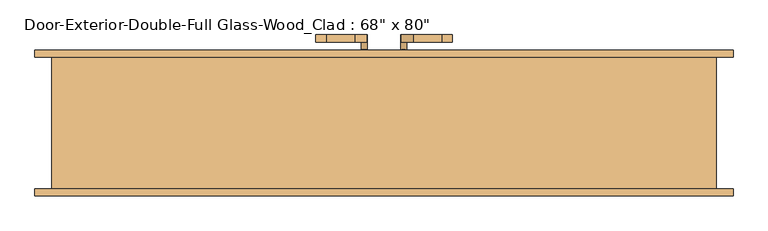
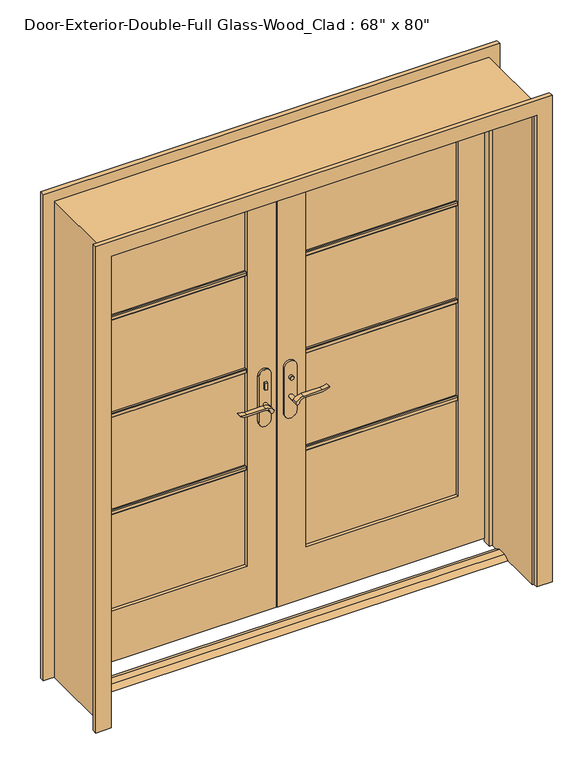
"""IFC4 building model written with IfcOpenShell, lengths in millimetres: door geometry."""

import ifcopenshell
import ifcopenshell.guid

model = None  # the IFC model being written
_history = None  # IfcOwnerHistory: only IFC2X3 demands one
_inside = {}  # id of a spatial element -> (the spatial element, [elements in it])
_under = {}  # id of a project, library or spatial element -> (it, [spatial elements below it])
_declared = {}  # id of a project -> (the project, [libraries it declares])
_typed = {}  # id of a type object -> (the type object, [elements of that type])
_made_of = {}  # id of a material, layer set ... -> (it, [elements and type objects made of it])


def new_model(schema):
    """Start an empty IFC model of exactly this schema.

    Asked for "IFC4X3", IfcOpenShell would pick the latest addendum, in which some entities
    have other attributes; the version numbers below select the first issue.
    IFC2X3 requires an IfcOwnerHistory on every rooted entity: one is made here for all.
    """
    global model, _history
    if schema == "IFC4X3":
        model = ifcopenshell.file(schema_version=(4, 3, 0, 0))
    else:
        model = ifcopenshell.file(schema=schema)
    _inside.clear()
    _under.clear()
    _declared.clear()
    _typed.clear()
    _made_of.clear()
    _history = None
    if model.schema == "IFC2X3":
        org = make("IfcOrganization", Name="unknown")
        user = make(
            "IfcPersonAndOrganization",
            ThePerson=make("IfcPerson", FamilyName="unknown"),
            TheOrganization=org,
        )
        app = make(
            "IfcApplication",
            ApplicationDeveloper=org,
            Version="unknown",
            ApplicationFullName="unknown",
            ApplicationIdentifier="unknown",
        )
        _history = make(
            "IfcOwnerHistory",
            OwningUser=user,
            OwningApplication=app,
            ChangeAction="ADDED",
            CreationDate=0,
        )
    return model


def make(cls, **values):
    """One entity of the class cls with the attributes given. An attribute that is None is left unset."""
    return model.create_entity(
        cls, **{name: value for name, value in values.items() if value is not None}
    )


def rooted(cls, **values):
    """An entity with a GlobalId (a new one), such as an element, a storey or a relation."""
    return make(cls, GlobalId=ifcopenshell.guid.new(), OwnerHistory=_history, **values)


def si_unit(unit_type, name, prefix=None):
    """IfcSIUnit, for example si_unit("LENGTHUNIT", "METRE", prefix="MILLI")."""
    return make("IfcSIUnit", UnitType=unit_type, Prefix=prefix, Name=name)


def assignment(units):
    """IfcUnitAssignment: the units of a project."""
    return None if units is None else make("IfcUnitAssignment", Units=units)


def point(xyz):
    """IfcCartesianPoint."""
    return None if xyz is None else make("IfcCartesianPoint", Coordinates=xyz)


def direction(xyz):
    """IfcDirection."""
    return None if xyz is None else make("IfcDirection", DirectionRatios=xyz)


def frame(location, z_axis=None, x_axis=None):
    """IfcAxis2Placement3D, a coordinate frame: its origin and axes. An axis left out is left unset."""
    return make(
        "IfcAxis2Placement3D",
        Location=point(location),
        Axis=direction(z_axis),
        RefDirection=direction(x_axis),
    )


def frame_2d(location, x_axis=None):
    """IfcAxis2Placement2D, a coordinate frame in the plane: its origin and x axis."""
    return make(
        "IfcAxis2Placement2D", Location=point(location), RefDirection=direction(x_axis)
    )


def origin():
    """The frame at (0, 0, 0) with its axes left unset."""
    return frame((0.0, 0.0, 0.0))


def place(relative_to, where):
    """IfcLocalPlacement: puts the frame where relative to a parent placement (None: the world)."""
    return make(
        "IfcLocalPlacement", PlacementRelTo=relative_to, RelativePlacement=where
    )


def context(
    kind, dimensions, precision=None, world=None, true_north=None, identifier=None
):
    """IfcGeometricRepresentationContext, for example the 3D "Model" context."""
    return make(
        "IfcGeometricRepresentationContext",
        ContextIdentifier=identifier,
        ContextType=kind,
        CoordinateSpaceDimension=dimensions,
        Precision=precision,
        WorldCoordinateSystem=world,
        TrueNorth=true_north,
    )


def project(units=None, contexts=None):
    """IfcProject with its units and contexts."""
    return rooted(
        "IfcProject",
        Name="project",
        RepresentationContexts=contexts,
        UnitsInContext=assignment(units),
    )


def spatial(cls, under=None, at=None, **own):
    """A site, building, storey or space (cls), placed at a placement, below another one or the project."""
    s = rooted(cls, ObjectPlacement=at, **own)
    if under is not None:
        _under.setdefault(under.id(), (under, []))[1].append(s)
    return s


def polyline(points):
    """IfcPolyline through the points."""
    return make("IfcPolyline", Points=[point(p) for p in points])


def circle_curve(where, radius):
    """IfcCircle in the frame where."""
    return make("IfcCircle", Position=where, Radius=radius)


def trimmed(basis, trim1, trim2, sense, master):
    """IfcTrimmedCurve: the piece of a basis curve between two trims."""
    return make(
        "IfcTrimmedCurve",
        BasisCurve=basis,
        Trim1=trim1,
        Trim2=trim2,
        SenseAgreement=sense,
        MasterRepresentation=master,
    )


def segment(curve, same_sense, transition):
    """IfcCompositeCurveSegment."""
    return make(
        "IfcCompositeCurveSegment",
        Transition=transition,
        SameSense=same_sense,
        ParentCurve=curve,
    )


def composite_curve(segments, self_intersect=None):
    """IfcCompositeCurve: segments joined end to end."""
    return make("IfcCompositeCurve", Segments=segments, SelfIntersect=self_intersect)


def outline(outer, holes=None, kind="AREA"):
    """IfcArbitraryClosedProfileDef: a profile drawn as a closed curve; with holes, ...WithVoids."""
    if holes is None:
        return make("IfcArbitraryClosedProfileDef", ProfileType=kind, OuterCurve=outer)
    return make(
        "IfcArbitraryProfileDefWithVoids",
        ProfileType=kind,
        OuterCurve=outer,
        InnerCurves=holes,
    )


def extrude(swept, where, along, depth):
    """IfcExtrudedAreaSolid: the profile swept, set in the frame where, extruded along a direction by depth."""
    return make(
        "IfcExtrudedAreaSolid",
        SweptArea=swept,
        Position=where,
        ExtrudedDirection=direction(along),
        Depth=depth,
    )


def faces_of(points, faces, orient=None, outer=None):
    """IfcFace entities. A face is a list of loops; a loop is a list of indices into points, from 0.

    orient and outer hold one flag for each loop. By default every Orientation is true, the
    first loop of a face is its IfcFaceOuterBound and the others are IfcFaceBound.
    """
    made = []
    for i, loops in enumerate(faces):
        bounds = []
        for j, loop in enumerate(loops):
            is_outer = j == 0 if outer is None else outer[i][j]
            bounds.append(
                make(
                    "IfcFaceOuterBound" if is_outer else "IfcFaceBound",
                    Bound=make("IfcPolyLoop", Polygon=[points[k] for k in loop]),
                    Orientation=True if orient is None else orient[i][j],
                )
            )
        made.append(make("IfcFace", Bounds=bounds))
    return made


def faceted_brep(points, faces, orient=None, outer=None, voids=None):
    """IfcFacetedBrep: a solid bounded by flat faces; with voids (closed shells), ...WithVoids."""
    shared = [point(p) for p in points]
    hull = make("IfcClosedShell", CfsFaces=faces_of(shared, faces, orient, outer))
    if voids is None:
        return make("IfcFacetedBrep", Outer=hull)
    return make(
        "IfcFacetedBrepWithVoids",
        Outer=hull,
        Voids=[
            make(cls, CfsFaces=faces_of(shared, fs, o, b)) for cls, fs, o, b in voids
        ],
    )


def shape(context_of_items, identifier, shape_type, items):
    """IfcShapeRepresentation: the items that make up one representation, for example the "Body"."""
    return make(
        "IfcShapeRepresentation",
        ContextOfItems=context_of_items,
        RepresentationIdentifier=identifier,
        RepresentationType=shape_type,
        Items=items,
    )


def source(mapping_origin, context_of_items, identifier, shape_type, items):
    """IfcRepresentationMap: a shape defined once, which mapped items show again and again."""
    return make(
        "IfcRepresentationMap",
        MappingOrigin=mapping_origin,
        MappedRepresentation=shape(context_of_items, identifier, shape_type, items),
    )


def transform(
    local_origin,
    x_axis=None,
    y_axis=None,
    z_axis=None,
    scale=None,
    scale2=None,
    scale3=None,
    uniform=True,
):
    """IfcCartesianTransformationOperator3D, or its non-uniform kind. x_axis, y_axis, z_axis: its Axis1, 2, 3."""
    if uniform:
        return make(
            "IfcCartesianTransformationOperator3D",
            Axis1=direction(x_axis),
            Axis2=direction(y_axis),
            LocalOrigin=point(local_origin),
            Scale=scale,
            Axis3=direction(z_axis),
        )
    return make(
        "IfcCartesianTransformationOperator3DnonUniform",
        Axis1=direction(x_axis),
        Axis2=direction(y_axis),
        LocalOrigin=point(local_origin),
        Scale=scale,
        Axis3=direction(z_axis),
        Scale2=scale2,
        Scale3=scale3,
    )


def mapped(mapping_source, mapping_target):
    """IfcMappedItem: shows the shape of a source again, moved by a transform."""
    return make(
        "IfcMappedItem", MappingSource=mapping_source, MappingTarget=mapping_target
    )


def made_of(thing, what):
    """Note that an element or type object is made of a material, layer set ...; save() writes the relation."""
    if what is not None:
        _made_of.setdefault(what.id(), (what, []))[1].append(thing)
    return thing


def element(
    cls,
    number,
    at=None,
    inside=None,
    cuts=None,
    type_object=None,
    material=None,
    context=None,
    identifier="Body",
    shape_type=None,
    held_by="IfcProductDefinitionShape",
    body=None,
    shapes=None,
    **own,
):
    """One element of the class cls, such as IfcWall. Its Tag is "e" and its number.

    at: its placement. inside: the storey or other place that contains it. cuts: it is an
    opening in that element (IfcRelVoidsElement). A single representation is given by context,
    identifier, shape_type and body (its items); several are given by shapes. held_by: the class
    of the entity that holds the representations. save() writes the other relations.
    """
    e = rooted(cls, Tag="e%d" % number, ObjectPlacement=at, **own)
    if body is not None:
        shapes = [shape(context, identifier, shape_type, body)]
    if shapes is not None:
        e.Representation = make(held_by, Representations=shapes)
    if inside is not None:
        _inside.setdefault(inside.id(), (inside, []))[1].append(e)
    if cuts is not None:
        rooted(
            "IfcRelVoidsElement", RelatingBuildingElement=cuts, RelatedOpeningElement=e
        )
    if type_object is not None:
        _typed.setdefault(type_object.id(), (type_object, []))[1].append(e)
    return made_of(e, material)


def aggregate(whole, parts):
    """IfcRelAggregates: a whole, such as a stair, and the parts it consists of."""
    return rooted("IfcRelAggregates", RelatingObject=whole, RelatedObjects=parts)


def save(model, path):
    """Write the relations noted so far, then the file.

    IfcRelAggregates (storeys below a building ...), IfcRelContainedInSpatialStructure (elements
    in a storey), IfcRelDefinesByType, IfcRelAssociatesMaterial and IfcRelDeclares: one each for
    every whole, place, type object, material and project.
    """
    for whole, parts in _under.values():
        aggregate(whole, parts)
    for where, things in _inside.values():
        rooted(
            "IfcRelContainedInSpatialStructure",
            RelatedElements=things,
            RelatingStructure=where,
        )
    for kind, things in _typed.values():
        rooted("IfcRelDefinesByType", RelatedObjects=things, RelatingType=kind)
    for what, things in _made_of.values():
        rooted("IfcRelAssociatesMaterial", RelatedObjects=things, RelatingMaterial=what)
    for by, libraries in _declared.values():
        rooted("IfcRelDeclares", RelatingContext=by, RelatedDefinitions=libraries)
    model.write(path)


def door_e0419d21(model_context):
    return source(origin(), model_context, "Body", "SolidModel", [
        extrude(outline(polyline([(19.05, 12.7), (53.975, 12.7), (79.375, 0.0), (-6.35, 0.0), (19.05, 12.7)])), frame((-863.6, 0.0, 0.0), z_axis=(1.0, 0.0, 0.0), x_axis=(0.0, 1.0, 0.0)), (0.0, 0.0, 1.0), 1727.2),
        extrude(outline(polyline([(-47.4019111, 118.1125), (-57.4019111, 118.1125), (-57.4019111, 128.1125), (-47.4019111, 128.1125), (-47.4019111, 118.1125)])), frame((0.0, 0.0, 981.9), z_axis=(0.0, 0.0, 1.0), x_axis=(1.0, 0.0, 0.0)), (0.0, 0.0, 1.0), 30.0),
        extrude(outline(composite_curve([segment(trimmed(circle_curve(frame_2d((996.9, -52.4019111)), 8.0), [point((996.9, -60.4019111))], [point((996.9, -44.4019111))], False, "CARTESIAN"), True, "CONTINUOUS"), segment(trimmed(circle_curve(frame_2d((996.9, -52.4019111)), 8.0), [point((996.9, -44.4019111))], [point((996.9, -60.4019111))], False, "CARTESIAN"), True, "CONTINUOUS")], self_intersect=False)), frame((0.0, 183.0375, 0.0), z_axis=(0.0, 1.0, 0.0), x_axis=(0.0, 0.0, 1.0)), (0.0, 0.0, 1.0), 10.0),
        extrude(outline(composite_curve([segment(trimmed(circle_curve(frame_2d((897.1555521, -76.0694241)), 37.2832219), [point((919.0523287, -45.8937749))], [point((934.4, -77.7693445))], False, "CARTESIAN"), True, "CONTINUOUS"), segment(polyline([(934.4, -77.7693445), (934.4, -154.045502)]), True, "CONTINUOUS"), segment(trimmed(circle_curve(frame_2d((1017.6850638, -153.9791202)), 83.2850902), [point((934.4, -154.045502))], [point((939.4, -182.4019111))], True, "CARTESIAN"), True, "CONTINUOUS"), segment(polyline([(939.4, -182.4019111), (936.6135558, -182.4019111)]), True, "CONTINUOUS"), segment(trimmed(circle_curve(frame_2d((986.6709207, -150.4622499)), 59.3791355), [point((936.6135558, -182.4019111))], [point((927.4, -154.045502))], False, "CARTESIAN"), True, "CONTINUOUS"), segment(polyline([(927.4, -154.045502), (927.4, -77.7881013)]), True, "CONTINUOUS"), segment(trimmed(circle_curve(frame_2d((909.2738613, -77.7881013)), 18.1261387), [point((927.4, -77.7881013))], [point((914.4, -60.4019111))], True, "CARTESIAN"), True, "CONTINUOUS"), segment(trimmed(circle_curve(frame_2d((914.4, -52.4019111)), 8.0), [point((914.4, -60.4019111))], [point((919.0523287, -45.8937749))], False, "CARTESIAN"), True, "CONTINUOUS")], self_intersect=False)), frame((0.0, 78.1125, 0.0), z_axis=(0.0, 1.0, 0.0), x_axis=(0.0, 0.0, 1.0)), (0.0, 0.0, 1.0), 20.0),
        extrude(outline(composite_curve([segment(trimmed(circle_curve(frame_2d((914.4, -52.4019111)), 8.0), [point((914.3999903, -60.4019111))], [point((919.0523287, -45.8937749))], False, "CARTESIAN"), True, "CONTINUOUS"), segment(trimmed(circle_curve(frame_2d((897.1555521, -76.0694241)), 37.2832219), [point((919.0523287, -45.8937749))], [point((934.4, -77.7693445))], False, "CARTESIAN"), True, "CONTINUOUS"), segment(polyline([(934.4, -77.7693445), (934.4, -154.045502)]), True, "CONTINUOUS"), segment(trimmed(circle_curve(frame_2d((1017.6850638, -153.9791202)), 83.2850902), [point((934.4, -154.045502))], [point((939.4, -182.4019111))], True, "CARTESIAN"), True, "CONTINUOUS"), segment(polyline([(939.4, -182.4019111), (936.6135558, -182.4019111)]), True, "CONTINUOUS"), segment(trimmed(circle_curve(frame_2d((986.6709207, -150.4622499)), 59.3791355), [point((936.6135558, -182.4019111))], [point((927.4, -154.045502))], False, "CARTESIAN"), True, "CONTINUOUS"), segment(polyline([(927.4, -154.045502), (927.4, -77.788099)]), True, "CONTINUOUS"), segment(trimmed(circle_curve(frame_2d((909.2738682, -77.788099)), 18.1261318), [point((927.4, -77.788099))], [point((914.3999903, -60.4019111))], True, "CARTESIAN"), True, "CONTINUOUS")], self_intersect=False)), frame((0.0, 213.0375, 0.0), z_axis=(0.0, 1.0, 0.0), x_axis=(0.0, 0.0, 1.0)), (0.0, 0.0, 1.0), 20.0),
        extrude(outline(composite_curve([segment(trimmed(circle_curve(frame_2d((914.4, -52.4019111)), 8.0), [point((914.4, -60.4019111))], [point((914.4, -44.4019111))], False, "CARTESIAN"), True, "CONTINUOUS"), segment(trimmed(circle_curve(frame_2d((914.4, -52.4019111)), 8.0), [point((914.4, -44.4019111))], [point((914.4, -60.4019111))], False, "CARTESIAN"), True, "CONTINUOUS")], self_intersect=False)), frame((0.0, 98.1125, 0.0), z_axis=(0.0, 1.0, 0.0), x_axis=(0.0, 0.0, 1.0)), (0.0, 0.0, 1.0), 30.0),
        extrude(outline(composite_curve([segment(trimmed(circle_curve(frame_2d((914.4, -52.4019111)), 8.0), [point((914.4, -60.4019111))], [point((914.4, -44.4019111))], False, "CARTESIAN"), True, "CONTINUOUS"), segment(trimmed(circle_curve(frame_2d((914.4, -52.4019111)), 8.0), [point((914.4, -44.4019111))], [point((914.4, -60.4019111))], False, "CARTESIAN"), True, "CONTINUOUS")], self_intersect=False)), frame((0.0, 183.0375, 0.0), z_axis=(0.0, 1.0, 0.0), x_axis=(0.0, 0.0, 1.0)), (0.0, 0.0, 1.0), 30.0),
        extrude(outline(composite_curve([segment(polyline([(844.4, -27.4019111), (1039.4, -27.4019111)]), True, "CONTINUOUS"), segment(trimmed(circle_curve(frame_2d((1039.4, -52.4019111)), 25.0), [point((1039.4, -27.4019111))], [point((1039.4, -77.4019111))], False, "CARTESIAN"), True, "CONTINUOUS"), segment(polyline([(1039.4, -77.4019111), (844.4, -77.4019111)]), True, "CONTINUOUS"), segment(trimmed(circle_curve(frame_2d((844.4, -52.4019111)), 25.0), [point((844.4, -77.4019111))], [point((844.4, -27.4019111))], False, "CARTESIAN"), True, "CONTINUOUS")], self_intersect=False)), frame((0.0, 128.1125, 0.0), z_axis=(0.0, 1.0, 0.0), x_axis=(0.0, 0.0, 1.0)), (0.0, 0.0, 1.0), 10.0),
        extrude(outline(composite_curve([segment(polyline([(844.4, -27.4019111), (1039.4, -27.4019111)]), True, "CONTINUOUS"), segment(trimmed(circle_curve(frame_2d((1039.4, -52.4019111)), 25.0), [point((1039.4, -27.4019111))], [point((1039.4, -77.4019111))], False, "CARTESIAN"), True, "CONTINUOUS"), segment(polyline([(1039.4, -77.4019111), (844.4, -77.4019111)]), True, "CONTINUOUS"), segment(trimmed(circle_curve(frame_2d((844.4, -52.4019111)), 25.0), [point((844.4, -77.4019111))], [point((844.4, -27.4019111))], False, "CARTESIAN"), True, "CONTINUOUS")], self_intersect=False)), frame((0.0, 173.0375, 0.0), z_axis=(0.0, 1.0, 0.0), x_axis=(0.0, 0.0, 1.0)), (0.0, 0.0, 1.0), 10.0),
        extrude(outline(polyline([(47.3875, 193.0375), (57.3875, 193.0375), (57.3875, 183.0375), (47.3875, 183.0375), (47.3875, 193.0375)])), frame((0.0, 0.0, 981.9), z_axis=(0.0, 0.0, 1.0), x_axis=(1.0, 0.0, 0.0)), (0.0, 0.0, 1.0), 30.0),
        extrude(outline(composite_curve([segment(trimmed(circle_curve(frame_2d((996.9, 52.3875)), 8.0), [point((996.9, 60.3875))], [point((996.9, 44.3875))], False, "CARTESIAN"), True, "CONTINUOUS"), segment(trimmed(circle_curve(frame_2d((996.9, 52.3875)), 8.0), [point((996.9, 44.3875))], [point((996.9, 60.3875))], False, "CARTESIAN"), True, "CONTINUOUS")], self_intersect=False)), frame((0.0, 118.1125, 0.0), z_axis=(0.0, 1.0, 0.0), x_axis=(0.0, 0.0, 1.0)), (0.0, 0.0, 1.0), 10.0),
        extrude(outline(composite_curve([segment(trimmed(circle_curve(frame_2d((914.4, 52.3875)), 8.0), [point((919.0523287, 45.8793637))], [point((914.4, 60.3875))], False, "CARTESIAN"), True, "CONTINUOUS"), segment(trimmed(circle_curve(frame_2d((909.2738613, 77.7736901)), 18.1261387), [point((914.4, 60.3875))], [point((927.4, 77.7736901))], True, "CARTESIAN"), True, "CONTINUOUS"), segment(polyline([(927.4, 77.7736901), (927.4, 154.0310909)]), True, "CONTINUOUS"), segment(trimmed(circle_curve(frame_2d((986.6709207, 150.4478388)), 59.3791355), [point((927.4, 154.0310909))], [point((936.6135558, 182.3875))], False, "CARTESIAN"), True, "CONTINUOUS"), segment(polyline([(936.6135558, 182.3875), (939.4, 182.3875)]), True, "CONTINUOUS"), segment(trimmed(circle_curve(frame_2d((1017.6850638, 153.9647091)), 83.2850902), [point((939.4, 182.3875))], [point((934.4, 154.0310909))], True, "CARTESIAN"), True, "CONTINUOUS"), segment(polyline([(934.4, 154.0310909), (934.4, 77.7549333)]), True, "CONTINUOUS"), segment(trimmed(circle_curve(frame_2d((897.1555521, 76.0550129)), 37.2832219), [point((934.4, 77.7549333))], [point((919.0523287, 45.8793637))], False, "CARTESIAN"), True, "CONTINUOUS")], self_intersect=False)), frame((0.0, 213.0375, 0.0), z_axis=(0.0, 1.0, 0.0), x_axis=(0.0, 0.0, 1.0)), (0.0, 0.0, 1.0), 20.0),
        extrude(outline(composite_curve([segment(trimmed(circle_curve(frame_2d((909.2738682, 77.7736878)), 18.1261318), [point((914.3999903, 60.3875))], [point((927.4, 77.7736878))], True, "CARTESIAN"), True, "CONTINUOUS"), segment(polyline([(927.4, 77.7736878), (927.4, 154.0310909)]), True, "CONTINUOUS"), segment(trimmed(circle_curve(frame_2d((986.6709207, 150.4478388)), 59.3791355), [point((927.4, 154.0310909))], [point((936.6135558, 182.3875))], False, "CARTESIAN"), True, "CONTINUOUS"), segment(polyline([(936.6135558, 182.3875), (939.4, 182.3875)]), True, "CONTINUOUS"), segment(trimmed(circle_curve(frame_2d((1017.6850638, 153.9647091)), 83.2850902), [point((939.4, 182.3875))], [point((934.4, 154.0310909))], True, "CARTESIAN"), True, "CONTINUOUS"), segment(polyline([(934.4, 154.0310909), (934.4, 77.7549333)]), True, "CONTINUOUS"), segment(trimmed(circle_curve(frame_2d((897.1555521, 76.0550129)), 37.2832219), [point((934.4, 77.7549333))], [point((919.0523287, 45.8793637))], False, "CARTESIAN"), True, "CONTINUOUS"), segment(trimmed(circle_curve(frame_2d((914.4, 52.3875)), 8.0), [point((919.0523287, 45.8793637))], [point((914.3999903, 60.3875))], False, "CARTESIAN"), True, "CONTINUOUS")], self_intersect=False)), frame((0.0, 78.1125, 0.0), z_axis=(0.0, 1.0, 0.0), x_axis=(0.0, 0.0, 1.0)), (0.0, 0.0, 1.0), 20.0),
        extrude(outline(composite_curve([segment(trimmed(circle_curve(frame_2d((914.4, 52.3875)), 8.0), [point((914.4, 60.3875))], [point((914.4, 44.3875))], False, "CARTESIAN"), True, "CONTINUOUS"), segment(trimmed(circle_curve(frame_2d((914.4, 52.3875)), 8.0), [point((914.4, 44.3875))], [point((914.4, 60.3875))], False, "CARTESIAN"), True, "CONTINUOUS")], self_intersect=False)), frame((0.0, 183.0375, 0.0), z_axis=(0.0, 1.0, 0.0), x_axis=(0.0, 0.0, 1.0)), (0.0, 0.0, 1.0), 30.0),
        extrude(outline(composite_curve([segment(trimmed(circle_curve(frame_2d((914.4, 52.3875)), 8.0), [point((914.4, 60.3875))], [point((914.4, 44.3875))], False, "CARTESIAN"), True, "CONTINUOUS"), segment(trimmed(circle_curve(frame_2d((914.4, 52.3875)), 8.0), [point((914.4, 44.3875))], [point((914.4, 60.3875))], False, "CARTESIAN"), True, "CONTINUOUS")], self_intersect=False)), frame((0.0, 98.1125, 0.0), z_axis=(0.0, 1.0, 0.0), x_axis=(0.0, 0.0, 1.0)), (0.0, 0.0, 1.0), 30.0),
        extrude(outline(composite_curve([segment(trimmed(circle_curve(frame_2d((844.4, 52.3875)), 25.0), [point((844.4, 27.3875))], [point((844.4, 77.3875))], False, "CARTESIAN"), True, "CONTINUOUS"), segment(polyline([(844.4, 77.3875), (1039.4, 77.3875)]), True, "CONTINUOUS"), segment(trimmed(circle_curve(frame_2d((1039.4, 52.3875)), 25.0), [point((1039.4, 77.3875))], [point((1039.4, 27.3875))], False, "CARTESIAN"), True, "CONTINUOUS"), segment(polyline([(1039.4, 27.3875), (844.4, 27.3875)]), True, "CONTINUOUS")], self_intersect=False)), frame((0.0, 173.0375, 0.0), z_axis=(0.0, 1.0, 0.0), x_axis=(0.0, 0.0, 1.0)), (0.0, 0.0, 1.0), 10.0),
        extrude(outline(composite_curve([segment(trimmed(circle_curve(frame_2d((844.4, 52.3875)), 25.0), [point((844.4, 27.3875))], [point((844.4, 77.3875))], False, "CARTESIAN"), True, "CONTINUOUS"), segment(polyline([(844.4, 77.3875), (1039.4, 77.3875)]), True, "CONTINUOUS"), segment(trimmed(circle_curve(frame_2d((1039.4, 52.3875)), 25.0), [point((1039.4, 77.3875))], [point((1039.4, 27.3875))], False, "CARTESIAN"), True, "CONTINUOUS"), segment(polyline([(1039.4, 27.3875), (844.4, 27.3875)]), True, "CONTINUOUS")], self_intersect=False)), frame((0.0, 128.1125, 0.0), z_axis=(0.0, 1.0, 0.0), x_axis=(0.0, 0.0, 1.0)), (0.0, 0.0, 1.0), 10.0),
        extrude(outline(polyline([(152.0825, 1502.171875), (152.0825, 1483.121875), (145.7325, 1483.121875), (142.5575, 1486.296875), (142.5575, 1498.996875), (145.7325, 1502.171875), (152.0825, 1502.171875)])), frame((120.65, 0.0, 0.0), z_axis=(1.0, 0.0, 0.0), x_axis=(0.0, 1.0, 0.0)), (0.0, 0.0, 1.0), 622.3),
        extrude(outline(polyline([(152.0825, 1081.88125), (152.0825, 1062.83125), (145.7325, 1062.83125), (142.5575, 1066.00625), (142.5575, 1078.70625), (145.7325, 1081.88125), (152.0825, 1081.88125)])), frame((120.65, 0.0, 0.0), z_axis=(1.0, 0.0, 0.0), x_axis=(0.0, 1.0, 0.0)), (0.0, 0.0, 1.0), 622.3),
        extrude(outline(polyline([(152.0825, 661.590625), (152.0825, 642.540625), (145.7325, 642.540625), (142.5575, 645.715625), (142.5575, 658.415625), (145.7325, 661.590625), (152.0825, 661.590625)])), frame((120.65, 0.0, 0.0), z_axis=(1.0, 0.0, 0.0), x_axis=(0.0, 1.0, 0.0)), (0.0, 0.0, 1.0), 622.3),
        extrude(outline(polyline([(159.0675, 1502.171875), (165.4175, 1502.171875), (168.5925, 1498.996875), (168.5925, 1486.296875), (165.4175, 1483.121875), (159.0675, 1483.121875), (159.0675, 1502.171875)])), frame((-742.95, 0.0, 0.0), z_axis=(1.0, 0.0, 0.0), x_axis=(0.0, 1.0, 0.0)), (0.0, 0.0, 1.0), 622.3),
        extrude(outline(polyline([(159.0675, 1081.88125), (165.4175, 1081.88125), (168.5925, 1078.70625), (168.5925, 1066.00625), (165.4175, 1062.83125), (159.0675, 1062.83125), (159.0675, 1081.88125)])), frame((-742.95, 0.0, 0.0), z_axis=(1.0, 0.0, 0.0), x_axis=(0.0, 1.0, 0.0)), (0.0, 0.0, 1.0), 622.3),
        extrude(outline(polyline([(159.0675, 661.590625), (165.4175, 661.590625), (168.5925, 658.415625), (168.5925, 645.715625), (165.4175, 642.540625), (159.0675, 642.540625), (159.0675, 661.590625)])), frame((-742.95, 0.0, 0.0), z_axis=(1.0, 0.0, 0.0), x_axis=(0.0, 1.0, 0.0)), (0.0, 0.0, 1.0), 622.3),
        extrude(outline(polyline([(159.0675, 1502.171875), (165.4175, 1502.171875), (168.5925, 1498.996875), (168.5925, 1486.296875), (165.4175, 1483.121875), (159.0675, 1483.121875), (159.0675, 1502.171875)])), frame((120.65, 0.0, 0.0), z_axis=(1.0, 0.0, 0.0), x_axis=(0.0, 1.0, 0.0)), (0.0, 0.0, 1.0), 622.3),
        extrude(outline(polyline([(159.0675, 1081.88125), (165.4175, 1081.88125), (168.5925, 1078.70625), (168.5925, 1066.00625), (165.4175, 1062.83125), (159.0675, 1062.83125), (159.0675, 1081.88125)])), frame((120.65, 0.0, 0.0), z_axis=(1.0, 0.0, 0.0), x_axis=(0.0, 1.0, 0.0)), (0.0, 0.0, 1.0), 622.3),
        extrude(outline(polyline([(159.0675, 661.590625), (165.4175, 661.590625), (168.5925, 658.415625), (168.5925, 645.715625), (165.4175, 642.540625), (159.0675, 642.540625), (159.0675, 661.590625)])), frame((120.65, 0.0, 0.0), z_axis=(1.0, 0.0, 0.0), x_axis=(0.0, 1.0, 0.0)), (0.0, 0.0, 1.0), 622.3),
        extrude(outline(polyline([(152.0825, 1502.171875), (152.0825, 1483.121875), (145.7325, 1483.121875), (142.5575, 1486.296875), (142.5575, 1498.996875), (145.7325, 1502.171875), (152.0825, 1502.171875)])), frame((-742.95, 0.0, 0.0), z_axis=(1.0, 0.0, 0.0), x_axis=(0.0, 1.0, 0.0)), (0.0, 0.0, 1.0), 622.3),
        extrude(outline(polyline([(152.0825, 1081.88125), (152.0825, 1062.83125), (145.7325, 1062.83125), (142.5575, 1066.00625), (142.5575, 1078.70625), (145.7325, 1081.88125), (152.0825, 1081.88125)])), frame((-742.95, 0.0, 0.0), z_axis=(1.0, 0.0, 0.0), x_axis=(0.0, 1.0, 0.0)), (0.0, 0.0, 1.0), 622.3),
        extrude(outline(polyline([(152.0825, 661.590625), (152.0825, 642.540625), (145.7325, 642.540625), (142.5575, 645.715625), (142.5575, 658.415625), (145.7325, 661.590625), (152.0825, 661.590625)])), frame((-742.95, 0.0, 0.0), z_axis=(1.0, 0.0, 0.0), x_axis=(0.0, 1.0, 0.0)), (0.0, 0.0, 1.0), 622.3),
        extrude(outline(polyline([(0.0, 869.95), (0.0, 933.45), (2101.85, 933.45), (2101.85, -933.45), (0.0, -933.45), (0.0, -869.95), (2038.35, -869.95), (2038.35, 869.95), (0.0, 869.95)])), frame((0.0, 173.0375, 0.0), z_axis=(0.0, 1.0, 0.0), x_axis=(0.0, 0.0, 1.0)), (0.0, 0.0, 1.0), 19.05),
        extrude(outline(polyline([(0.0, 869.95), (0.0, 933.45), (2101.85, 933.45), (2101.85, -933.45), (0.0, -933.45), (0.0, -869.95), (2038.35, -869.95), (2038.35, 869.95), (0.0, 869.95)])), frame((0.0, -198.4375, 0.0), z_axis=(0.0, 1.0, 0.0), x_axis=(0.0, 0.0, 1.0)), (0.0, 0.0, 1.0), 19.05),
        extrude(outline(polyline([(12.7, 863.6), (2032.0, 863.6), (2032.0, 1.5875), (12.7, 1.5875), (12.7, 863.6)]), holes=[polyline([(1912.9375, 120.65), (1912.9375, 742.95), (231.775, 742.95), (231.775, 120.65), (1912.9375, 120.65)])]), frame((0.0, 138.1125, 0.0), z_axis=(0.0, 1.0, 0.0), x_axis=(0.0, 0.0, 1.0)), (0.0, 0.0, 1.0), 34.925),
        extrude(outline(polyline([(2032.0, -863.6), (12.7, -863.6), (12.7, -1.6019111), (2032.0, -1.6019111), (2032.0, -863.6)]), holes=[polyline([(231.775, -742.95), (1912.9375, -742.95), (1912.9375, -120.65), (231.775, -120.65), (231.775, -742.95)])]), frame((0.0, 138.1125, 0.0), z_axis=(0.0, 1.0, 0.0), x_axis=(0.0, 0.0, 1.0)), (0.0, 0.0, 1.0), 34.925),
        faceted_brep([(889.0, 173.0375, 0.0), (889.0, -179.3875, 0.0), (863.6, -179.3875, 0.0), (863.6, 103.1875, 0.0), (850.9, 103.1875, 0.0), (850.9, 138.1125, 0.0), (863.6, 138.1125, 0.0), (863.6, 173.0375, 0.0), (889.0, 173.0375, 2057.4), (889.0, -179.3875, 2057.4), (-889.0, -179.3875, 2057.4), (-889.0, -179.3875, 0.0), (-863.6, -179.3875, 0.0), (-863.6, -179.3875, 2032.0), (863.6, -179.3875, 2032.0), (863.6, 103.1875, 2032.0), (-863.6, 103.1875, 2032.0), (-863.6, 103.1875, 0.0), (-850.9, 103.1875, 0.0), (-850.9, 103.1875, 2019.3), (850.9, 103.1875, 2019.3), (850.9, 138.1125, 2019.3), (1.5875, 138.1125, 2019.3), (-1.6019111, 138.1125, 2019.3), (-850.9, 138.1125, 2019.3), (-850.9, 138.1125, 0.0), (-863.6, 138.1125, 0.0), (-863.6, 138.1125, 2032.0), (-1.6019111, 138.1125, 2032.0), (1.5875, 138.1125, 2032.0), (863.6, 138.1125, 2032.0), (863.6, 173.0375, 2032.0), (1.5875, 173.0375, 2032.0), (-1.6019111, 173.0375, 2032.0), (-863.6, 173.0375, 2032.0), (-863.6, 173.0375, 0.0), (-889.0, 173.0375, 0.0), (-889.0, 173.0375, 2057.4)], [[[0, 1, 2, 3, 4, 5, 6, 7]], [[1, 0, 8, 9]], [[2, 1, 9, 10, 11, 12, 13, 14]], [[3, 2, 14, 15]], [[4, 3, 15, 16, 17, 18, 19, 20]], [[5, 4, 20, 21]], [[6, 5, 21, 22, 23, 24, 25, 26, 27, 28, 29, 30]], [[7, 6, 30, 31]], [[0, 7, 31, 32, 33, 34, 35, 36, 37, 8]], [[9, 8, 37, 10]], [[14, 13, 16, 15]], [[20, 19, 24, 23, 22, 21]], [[31, 30, 29, 28, 27, 34, 33, 32]], [[12, 11, 36, 35, 26, 25, 18, 17]], [[11, 10, 37, 36]], [[13, 12, 17, 16]], [[19, 18, 25, 24]], [[27, 26, 35, 34]]]),
        extrude(outline(polyline([(742.95, 152.0825), (120.65, 152.0825), (120.65, 159.0675), (742.95, 159.0675), (742.95, 152.0825)])), frame((0.0, 0.0, 231.775), z_axis=(0.0, 0.0, 1.0), x_axis=(1.0, 0.0, 0.0)), (0.0, 0.0, 1.0), 1681.1625),
        extrude(outline(polyline([(-120.65, 152.0825), (-742.95, 152.0825), (-742.95, 159.0675), (-120.65, 159.0675), (-120.65, 152.0825)])), frame((0.0, 0.0, 231.775), z_axis=(0.0, 0.0, 1.0), x_axis=(1.0, 0.0, 0.0)), (0.0, 0.0, 1.0), 1681.1625),
    ])


if __name__ == "__main__":
    model = new_model("IFC4")
    model_context = context("Model", 3, world=origin())
    ifc_project = project(units=[si_unit("LENGTHUNIT", "METRE", prefix="MILLI")], contexts=[model_context])
    site = spatial("IfcSite", under=ifc_project)
    building = spatial("IfcBuilding", under=site)
    placement = place(None, origin())
    door_shape = door_e0419d21(model_context)
    element("IfcDoor", 1, ObjectType="Door-Exterior-Double-Full Glass-Wood_Clad : 68\" x 80\"", at=placement, inside=building, context=model_context, shape_type="MappedRepresentation", body=[
        mapped(door_shape, transform((0.0, 0.0, 0.0), x_axis=(1.0, 0.0, 0.0), y_axis=(0.0, 1.0, 0.0), z_axis=(0.0, 0.0, 1.0))),
    ])
    save(model, "model.ifc")

# Revit data of these elements
# Type "Door-Exterior-Double-Full Glass-Wood_Clad : 68\" x 80\""
#   Type Mark = "21"
#   Assembly Code = "B2030100"
#   Analytic Construction = "French door, wood frame with double glass"
#   Top Rail = 0' - 4 11/16"
#   Threshold Offset [instance default] = 0' - 0 1/2"
#   Thickness = 0' - 1 3/8"
#   Thermal Resistance (R) = 1.9158 (h·ft²·°F)/BTU
#   Swing Angle [instance default] = 90.0000°
#   Stiles = 0' - 4 3/4"
#   Rough Width = 5' - 10"
#   Rough Height = 6' - 9"
#   Panel Width = 2' - 10"
#   Door Offset [instance default] = 0' - 0"
#   Height = 6' - 8"
#   Width = 5' - 8"
#   Heat Transfer Coefficient (U) = 0.5220 BTU/(h·ft²·°F)
#   Bottom Rail = 0' - 9 1/8"
#   Exterior Trim [instance default] = yes
#   Threshold [instance default] = yes
#   Show Grill [instance default] = yes
#   Function = 1
#   Trim Material = Cherry
#   Threshold Material = Cherry
#   Panel Material = Cherry
#   Glazing = Glass
#   Frame Material = Cherry
#   Door Handle Material = Aluminum
#   Visual Light Transmittance = 0
#   Solar Heat Gain Coefficient = 0
#   Wall Closure = (empty or 0)
#   Construction Type = (empty or 0)
# Element 1 (IfcDoor, "Door-Exterior-Double-Full Glass-Wood_Clad : 68\" x 80\"")
#   Materials on its faces: "Cherry", "Aluminum", "Glass"
# Materials
#   "Cherry": class "Wood", colour RGB 226 177 128, transparency 0, Description = "Prunus Serotina", Cost = 0
#   "Glass": class "Glass", colour RGB 0 128 192, transparency 0.75, Description = "Soda Lime Glass", Cost = 0
#   "Aluminum": class "Metal", colour RGB 247 247 247, transparency 0, Description = "Aluminum 6061", Cost = 0
